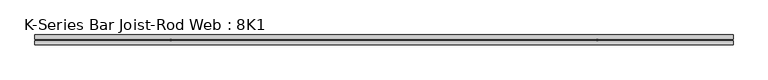
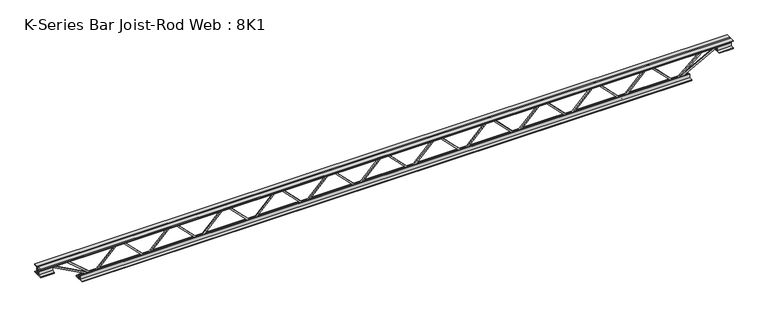
"""IFC4 building model written with IfcOpenShell, lengths in millimetres: beam geometry, K-Series Bar Joist-Rod Web : 8K1."""

from ifc_helpers import new_model, si_unit, frame, origin, place, context, project, spatial, polyline, outline, extrude, source, transform, mapped, element, save


def k_series_bar_joist_rod_web_8k1_fc2c6b5f(model_context):
    return source(origin(), model_context, "Body", "SweptSolid", [
        extrude(outline(polyline([(-90.4875, 1358.1275834), (-100.0125, 1358.1275834), (-100.0125, 1363.2961981), (90.4875, 1550.9644243), (90.4875, 1553.3271949), (-100.0125, 1740.9954211), (-100.0125, 1746.1640358), (-90.4875, 1746.1640358), (-90.4875, 1744.9826505), (100.0125, 1557.3144243), (100.0125, 1546.9771949), (-90.4875, 1359.3089687), (-90.4875, 1358.1275834)])), frame((0.0, -4.7625, 0.0), z_axis=(0.0, 1.0, 0.0), x_axis=(0.0, 0.0, 1.0)), (0.0, 0.0, 1.0), 9.525),
        extrude(outline(polyline([(-90.4875, 970.091131), (-100.0125, 970.091131), (-100.0125, 975.2597457), (90.4875, 1162.9279719), (90.4875, 1165.2907425), (-100.0125, 1352.9589687), (-100.0125, 1358.1275834), (-90.4875, 1358.1275834), (-90.4875, 1356.9461981), (100.0125, 1169.2779719), (100.0125, 1158.9407425), (-90.4875, 971.2725163), (-90.4875, 970.091131)])), frame((0.0, -4.7625, 0.0), z_axis=(0.0, 1.0, 0.0), x_axis=(0.0, 0.0, 1.0)), (0.0, 0.0, 1.0), 9.525),
        extrude(outline(polyline([(-90.4875, 582.0546786), (-100.0125, 582.0546786), (-100.0125, 587.2232933), (90.4875, 774.8915195), (90.4875, 777.2542901), (-100.0125, 964.9225163), (-100.0125, 970.091131), (-90.4875, 970.091131), (-90.4875, 968.9097457), (100.0125, 781.2415195), (100.0125, 770.9042901), (-90.4875, 583.2360639), (-90.4875, 582.0546786)])), frame((0.0, -4.7625, 0.0), z_axis=(0.0, 1.0, 0.0), x_axis=(0.0, 0.0, 1.0)), (0.0, 0.0, 1.0), 9.525),
        extrude(outline(polyline([(-90.4875, 194.0182262), (-100.0125, 194.0182262), (-100.0125, 199.1868409), (90.4875, 386.8550671), (90.4875, 389.2178377), (-100.0125, 576.8860639), (-100.0125, 582.0546786), (-90.4875, 582.0546786), (-90.4875, 580.8732933), (100.0125, 393.2050671), (100.0125, 382.8678377), (-90.4875, 195.1996115), (-90.4875, 194.0182262)])), frame((0.0, -4.7625, 0.0), z_axis=(0.0, 1.0, 0.0), x_axis=(0.0, 0.0, 1.0)), (0.0, 0.0, 1.0), 9.525),
        extrude(outline(polyline([(-90.4875, -194.0182262), (-100.0125, -194.0182262), (-100.0125, -188.8496115), (90.4875, -1.1813853), (90.4875, 1.1813853), (-100.0125, 188.8496115), (-100.0125, 194.0182262), (-90.4875, 194.0182262), (-90.4875, 192.8368409), (100.0125, 5.1686147), (100.0125, -5.1686147), (-90.4875, -192.8368409), (-90.4875, -194.0182262)])), frame((0.0, -4.7625, 0.0), z_axis=(0.0, 1.0, 0.0), x_axis=(0.0, 0.0, 1.0)), (0.0, 0.0, 1.0), 9.525),
        extrude(outline(polyline([(-90.4875, -582.0546786), (-100.0125, -582.0546786), (-100.0125, -576.8860639), (90.4875, -389.2178377), (90.4875, -386.8550671), (-100.0125, -199.1868409), (-100.0125, -194.0182262), (-90.4875, -194.0182262), (-90.4875, -195.1996115), (100.0125, -382.8678377), (100.0125, -393.2050671), (-90.4875, -580.8732933), (-90.4875, -582.0546786)])), frame((0.0, -4.7625, 0.0), z_axis=(0.0, 1.0, 0.0), x_axis=(0.0, 0.0, 1.0)), (0.0, 0.0, 1.0), 9.525),
        extrude(outline(polyline([(-90.4875, -970.091131), (-100.0125, -970.091131), (-100.0125, -964.9225163), (90.4875, -777.2542901), (90.4875, -774.8915195), (-100.0125, -587.2232933), (-100.0125, -582.0546786), (-90.4875, -582.0546786), (-90.4875, -583.2360639), (100.0125, -770.9042901), (100.0125, -781.2415195), (-90.4875, -968.9097457), (-90.4875, -970.091131)])), frame((0.0, -4.7625, 0.0), z_axis=(0.0, 1.0, 0.0), x_axis=(0.0, 0.0, 1.0)), (0.0, 0.0, 1.0), 9.525),
        extrude(outline(polyline([(-90.4875, -1358.1275834), (-100.0125, -1358.1275834), (-100.0125, -1352.9589687), (90.4875, -1165.2907425), (90.4875, -1162.9279719), (-100.0125, -975.2597457), (-100.0125, -970.091131), (-90.4875, -970.091131), (-90.4875, -971.2725163), (100.0125, -1158.9407425), (100.0125, -1169.2779719), (-90.4875, -1356.9461981), (-90.4875, -1358.1275834)])), frame((0.0, -4.7625, 0.0), z_axis=(0.0, 1.0, 0.0), x_axis=(0.0, 0.0, 1.0)), (0.0, 0.0, 1.0), 9.525),
        extrude(outline(polyline([(-90.4875, -1746.1640358), (-100.0125, -1746.1640358), (-100.0125, -1740.9954211), (90.4875, -1553.3271949), (90.4875, -1550.9644243), (-100.0125, -1363.2961981), (-100.0125, -1358.1275834), (-90.4875, -1358.1275834), (-90.4875, -1359.3089687), (100.0125, -1546.9771949), (100.0125, -1557.3144243), (-90.4875, -1744.9826505), (-90.4875, -1746.1640358)])), frame((0.0, -4.7625, 0.0), z_axis=(0.0, 1.0, 0.0), x_axis=(0.0, 0.0, 1.0)), (0.0, 0.0, 1.0), 9.525),
        extrude(outline(polyline([(-90.4875, 1746.1640358), (-100.0125, 1746.1640358), (-100.0125, 1751.3326505), (90.4875, 1939.0008767), (90.4875, 1941.3636473), (-100.0125, 2129.0318735), (-100.0125, 2134.2004882), (-90.4875, 2134.2004882), (-90.4875, 2133.0191029), (100.0125, 1945.3508767), (100.0125, 1935.0136473), (-90.4875, 1747.3454211), (-90.4875, 1746.1640358)])), frame((0.0, -4.7625, 0.0), z_axis=(0.0, 1.0, 0.0), x_axis=(0.0, 0.0, 1.0)), (0.0, 0.0, 1.0), 9.525),
        extrude(outline(polyline([(-90.4875, -2134.2004882), (-100.0125, -2134.2004882), (-100.0125, -2129.0318735), (90.4875, -1941.3636473), (90.4875, -1939.0008767), (-100.0125, -1751.3326505), (-100.0125, -1746.1640358), (-90.4875, -1746.1640358), (-90.4875, -1747.3454211), (100.0125, -1935.0136473), (100.0125, -1945.3508767), (-90.4875, -2133.0191029), (-90.4875, -2134.2004882)])), frame((0.0, -4.7625, 0.0), z_axis=(0.0, 1.0, 0.0), x_axis=(0.0, 0.0, 1.0)), (0.0, 0.0, 1.0), 9.525),
        extrude(outline(polyline([(4.7625, 101.6), (36.5125, 101.6), (36.5125, 95.25), (11.1125, 95.25), (11.1125, 69.85), (4.7625, 69.85), (4.7625, 101.6)])), frame((-2540.6004882, 0.0, 0.0), z_axis=(1.0, 0.0, 0.0), x_axis=(0.0, 1.0, 0.0)), (0.0, 0.0, 1.0), 5081.2009764),
        extrude(outline(polyline([(-4.7625, 101.6), (-4.7625, 69.85), (-11.1125, 69.85), (-11.1125, 95.25), (-36.5125, 95.25), (-36.5125, 101.6), (-4.7625, 101.6)])), frame((-2540.6004882, 0.0, 0.0), z_axis=(1.0, 0.0, 0.0), x_axis=(0.0, 1.0, 0.0)), (0.0, 0.0, 1.0), 5081.2009764),
        extrude(outline(polyline([(-4.7625, 38.1), (-36.5125, 38.1), (-36.5125, 44.45), (-11.1125, 44.45), (-11.1125, 69.85), (-4.7625, 69.85), (-4.7625, 38.1)])), frame((-2540.6004882, 0.0, 0.0), z_axis=(1.0, 0.0, 0.0), x_axis=(0.0, 1.0, 0.0)), (0.0, 0.0, 1.0), 101.6),
        extrude(outline(polyline([(36.5125, 38.1), (4.7625, 38.1), (4.7625, 69.85), (11.1125, 69.85), (11.1125, 44.45), (36.5125, 44.45), (36.5125, 38.1)])), frame((-2540.6004882, 0.0, 0.0), z_axis=(1.0, 0.0, 0.0), x_axis=(0.0, 1.0, 0.0)), (0.0, 0.0, 1.0), 101.6),
        extrude(outline(polyline([(4.7625, 38.1), (4.7625, 69.85), (11.1125, 69.85), (11.1125, 44.45), (36.5125, 44.45), (36.5125, 38.1), (4.7625, 38.1)])), frame((2439.0004882, 0.0, 0.0), z_axis=(1.0, 0.0, 0.0), x_axis=(0.0, 1.0, 0.0)), (0.0, 0.0, 1.0), 101.6),
        extrude(outline(polyline([(-4.7625, 38.1), (-36.5125, 38.1), (-36.5125, 44.45), (-11.1125, 44.45), (-11.1125, 69.85), (-4.7625, 69.85), (-4.7625, 38.1)])), frame((2439.0004882, 0.0, 0.0), z_axis=(1.0, 0.0, 0.0), x_axis=(0.0, 1.0, 0.0)), (0.0, 0.0, 1.0), 101.6),
        extrude(outline(polyline([(4.7625, -101.6), (4.7625, -69.85), (11.1125, -69.85), (11.1125, -95.25), (36.5125, -95.25), (36.5125, -101.6), (4.7625, -101.6)])), frame((-2235.8004882, 0.0, 0.0), z_axis=(1.0, 0.0, 0.0), x_axis=(0.0, 1.0, 0.0)), (0.0, 0.0, 1.0), 4471.6009764),
        extrude(outline(polyline([(-4.7625, -101.6), (-36.5125, -101.6), (-36.5125, -95.25), (-11.1125, -95.25), (-11.1125, -69.85), (-4.7625, -69.85), (-4.7625, -101.6)])), frame((-2235.8004882, 0.0, 0.0), z_axis=(1.0, 0.0, 0.0), x_axis=(0.0, 1.0, 0.0)), (0.0, 0.0, 1.0), 4471.6009764),
        extrude(outline(polyline([(0.0, -9.525), (0.0, 0.0), (346.6425392, 0.0), (346.6425392, -9.525), (0.0, -9.525)])), frame((-2441.2687867, 4.7625, 65.662372), z_axis=(0.47628314854008114, 0.0, 0.8792919665371378), x_axis=(0.8792919665371378, 0.0, -0.47628314854008114)), (0.0, 0.0, 1.0), 9.525),
        extrude(outline(polyline([(0.0, -9.525), (0.0, 0.0), (254.7569079, 0.0), (254.7569079, -9.525), (0.0, -9.525)])), frame((-2331.305142, 4.7625, 66.2229666), z_axis=(0.6480687860160269, 0.0, 0.7615818068938578), x_axis=(0.7615818068938578, 0.0, -0.6480687860160269)), (0.0, 0.0, 1.0), 9.525),
        extrude(outline(polyline([(0.0, -9.525), (0.0, 0.0), (346.6425392, 0.0), (346.6425392, -9.525), (0.0, -9.525)])), frame((2441.2687867, -4.7625, 65.662372), z_axis=(-0.4762831485400423, 0.0, 0.8792919665371588), x_axis=(-0.8792919665371588, 0.0, -0.4762831485400423)), (0.0, 0.0, 1.0), 9.525),
        extrude(outline(polyline([(0.0, -9.525), (0.0, 0.0), (254.7569079, 0.0), (254.7569079, -9.525), (0.0, -9.525)])), frame((2331.305142, -4.7625, 66.2229666), z_axis=(-0.6480687860159982, 0.0, 0.7615818068938822), x_axis=(-0.7615818068938822, 0.0, -0.6480687860159982)), (0.0, 0.0, 1.0), 9.525),
    ])


if __name__ == "__main__":
    model = new_model("IFC4")
    model_context = context("Model", 3, world=origin())
    ifc_project = project(units=[si_unit("LENGTHUNIT", "METRE", prefix="MILLI")], contexts=[model_context])
    site = spatial("IfcSite", under=ifc_project)
    building = spatial("IfcBuilding", under=site)
    placement = place(None, origin())
    k_series_bar_joist_rod_web_8k1_shape = k_series_bar_joist_rod_web_8k1_fc2c6b5f(model_context)
    element("IfcBeam", 1, ObjectType="K-Series Bar Joist-Rod Web : 8K1", at=placement, inside=building, context=model_context, shape_type="MappedRepresentation", body=[
        mapped(k_series_bar_joist_rod_web_8k1_shape, transform((0.0, 0.0, 0.0), x_axis=(1.0, 0.0, 0.0), y_axis=(0.0, 1.0, 0.0), z_axis=(0.0, 0.0, 1.0))),
    ])
    save(model, "model.ifc")

# Revit data of these elements
# Type "K-Series Bar Joist-Rod Web : 8K1"
#   Assembly Code = "B1010350"
#   Wt = 5.1
#   Web Thickness = 0' - 0 3/8"
#   Start Offset [instance default] = 0' - 0"
#   Start Extension [instance default] = 0' - 0"
#   Seat Length = 0' - 4"
#   Seat Depth = 0' - 2 1/2"
#   PanelArrayLength [instance default] = 21' - 4"
#   Panel [instance default] = 1' - 4"
#   End Offset [instance default] = 0' - 0"
#   End Extension [instance default] = 0' - 0"
#   End Panel = 1' - 4"
#   Cord Leg = 0' - 1 1/4"
#   Chord Thickness = 0' - 0 1/4"
#   Length [instance default] = 24' - 0"
#   Depth = 0' - 8"
#   PanelArrayNum [instance default] = 16
#   Rendering Material = none
# Element 1 (IfcBeam, "K-Series Bar Joist-Rod Web : 8K1")
#   PanelArrayLength = 14' - 0.04728"
#   Panel = 1' - 3.27703"
#   PanelArrayNum = 11
